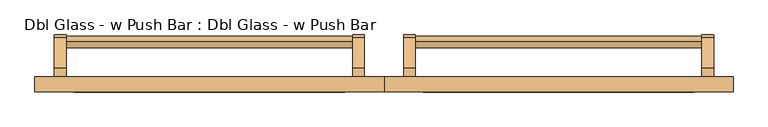
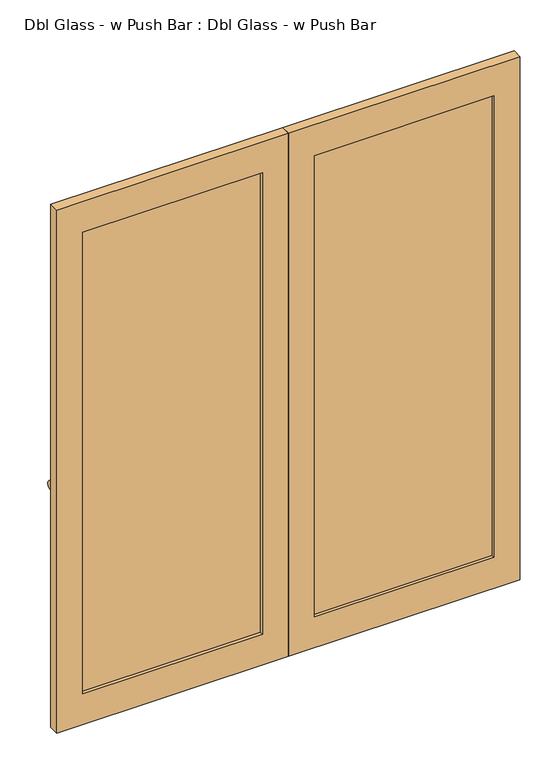
"""IFC4 building model written with IfcOpenShell, lengths in millimetres: door geometry, Dbl Glass - w Push Bar : Dbl Glass - w Push Bar."""

import ifcopenshell
import ifcopenshell.guid

model = None  # the IFC model being written
_history = None  # IfcOwnerHistory: only IFC2X3 demands one
_inside = {}  # id of a spatial element -> (the spatial element, [elements in it])
_under = {}  # id of a project, library or spatial element -> (it, [spatial elements below it])
_declared = {}  # id of a project -> (the project, [libraries it declares])
_typed = {}  # id of a type object -> (the type object, [elements of that type])
_made_of = {}  # id of a material, layer set ... -> (it, [elements and type objects made of it])


def new_model(schema):
    """Start an empty IFC model of exactly this schema.

    Asked for "IFC4X3", IfcOpenShell would pick the latest addendum, in which some entities
    have other attributes; the version numbers below select the first issue.
    IFC2X3 requires an IfcOwnerHistory on every rooted entity: one is made here for all.
    """
    global model, _history
    if schema == "IFC4X3":
        model = ifcopenshell.file(schema_version=(4, 3, 0, 0))
    else:
        model = ifcopenshell.file(schema=schema)
    _inside.clear()
    _under.clear()
    _declared.clear()
    _typed.clear()
    _made_of.clear()
    _history = None
    if model.schema == "IFC2X3":
        org = make("IfcOrganization", Name="unknown")
        user = make(
            "IfcPersonAndOrganization",
            ThePerson=make("IfcPerson", FamilyName="unknown"),
            TheOrganization=org,
        )
        app = make(
            "IfcApplication",
            ApplicationDeveloper=org,
            Version="unknown",
            ApplicationFullName="unknown",
            ApplicationIdentifier="unknown",
        )
        _history = make(
            "IfcOwnerHistory",
            OwningUser=user,
            OwningApplication=app,
            ChangeAction="ADDED",
            CreationDate=0,
        )
    return model


def make(cls, **values):
    """One entity of the class cls with the attributes given. An attribute that is None is left unset."""
    return model.create_entity(
        cls, **{name: value for name, value in values.items() if value is not None}
    )


def rooted(cls, **values):
    """An entity with a GlobalId (a new one), such as an element, a storey or a relation."""
    return make(cls, GlobalId=ifcopenshell.guid.new(), OwnerHistory=_history, **values)


def si_unit(unit_type, name, prefix=None):
    """IfcSIUnit, for example si_unit("LENGTHUNIT", "METRE", prefix="MILLI")."""
    return make("IfcSIUnit", UnitType=unit_type, Prefix=prefix, Name=name)


def assignment(units):
    """IfcUnitAssignment: the units of a project."""
    return None if units is None else make("IfcUnitAssignment", Units=units)


def point(xyz):
    """IfcCartesianPoint."""
    return None if xyz is None else make("IfcCartesianPoint", Coordinates=xyz)


def direction(xyz):
    """IfcDirection."""
    return None if xyz is None else make("IfcDirection", DirectionRatios=xyz)


def frame(location, z_axis=None, x_axis=None):
    """IfcAxis2Placement3D, a coordinate frame: its origin and axes. An axis left out is left unset."""
    return make(
        "IfcAxis2Placement3D",
        Location=point(location),
        Axis=direction(z_axis),
        RefDirection=direction(x_axis),
    )


def frame_2d(location, x_axis=None):
    """IfcAxis2Placement2D, a coordinate frame in the plane: its origin and x axis."""
    return make(
        "IfcAxis2Placement2D", Location=point(location), RefDirection=direction(x_axis)
    )


def origin():
    """The frame at (0, 0, 0) with its axes left unset."""
    return frame((0.0, 0.0, 0.0))


def place(relative_to, where):
    """IfcLocalPlacement: puts the frame where relative to a parent placement (None: the world)."""
    return make(
        "IfcLocalPlacement", PlacementRelTo=relative_to, RelativePlacement=where
    )


def context(
    kind, dimensions, precision=None, world=None, true_north=None, identifier=None
):
    """IfcGeometricRepresentationContext, for example the 3D "Model" context."""
    return make(
        "IfcGeometricRepresentationContext",
        ContextIdentifier=identifier,
        ContextType=kind,
        CoordinateSpaceDimension=dimensions,
        Precision=precision,
        WorldCoordinateSystem=world,
        TrueNorth=true_north,
    )


def project(units=None, contexts=None):
    """IfcProject with its units and contexts."""
    return rooted(
        "IfcProject",
        Name="project",
        RepresentationContexts=contexts,
        UnitsInContext=assignment(units),
    )


def spatial(cls, under=None, at=None, **own):
    """A site, building, storey or space (cls), placed at a placement, below another one or the project."""
    s = rooted(cls, ObjectPlacement=at, **own)
    if under is not None:
        _under.setdefault(under.id(), (under, []))[1].append(s)
    return s


def polyline(points):
    """IfcPolyline through the points."""
    return make("IfcPolyline", Points=[point(p) for p in points])


def circle_curve(where, radius):
    """IfcCircle in the frame where."""
    return make("IfcCircle", Position=where, Radius=radius)


def trimmed(basis, trim1, trim2, sense, master):
    """IfcTrimmedCurve: the piece of a basis curve between two trims."""
    return make(
        "IfcTrimmedCurve",
        BasisCurve=basis,
        Trim1=trim1,
        Trim2=trim2,
        SenseAgreement=sense,
        MasterRepresentation=master,
    )


def segment(curve, same_sense, transition):
    """IfcCompositeCurveSegment."""
    return make(
        "IfcCompositeCurveSegment",
        Transition=transition,
        SameSense=same_sense,
        ParentCurve=curve,
    )


def composite_curve(segments, self_intersect=None):
    """IfcCompositeCurve: segments joined end to end."""
    return make("IfcCompositeCurve", Segments=segments, SelfIntersect=self_intersect)


def outline(outer, holes=None, kind="AREA"):
    """IfcArbitraryClosedProfileDef: a profile drawn as a closed curve; with holes, ...WithVoids."""
    if holes is None:
        return make("IfcArbitraryClosedProfileDef", ProfileType=kind, OuterCurve=outer)
    return make(
        "IfcArbitraryProfileDefWithVoids",
        ProfileType=kind,
        OuterCurve=outer,
        InnerCurves=holes,
    )


def extrude(swept, where, along, depth):
    """IfcExtrudedAreaSolid: the profile swept, set in the frame where, extruded along a direction by depth."""
    return make(
        "IfcExtrudedAreaSolid",
        SweptArea=swept,
        Position=where,
        ExtrudedDirection=direction(along),
        Depth=depth,
    )


def shape(context_of_items, identifier, shape_type, items):
    """IfcShapeRepresentation: the items that make up one representation, for example the "Body"."""
    return make(
        "IfcShapeRepresentation",
        ContextOfItems=context_of_items,
        RepresentationIdentifier=identifier,
        RepresentationType=shape_type,
        Items=items,
    )


def source(mapping_origin, context_of_items, identifier, shape_type, items):
    """IfcRepresentationMap: a shape defined once, which mapped items show again and again."""
    return make(
        "IfcRepresentationMap",
        MappingOrigin=mapping_origin,
        MappedRepresentation=shape(context_of_items, identifier, shape_type, items),
    )


def transform(
    local_origin,
    x_axis=None,
    y_axis=None,
    z_axis=None,
    scale=None,
    scale2=None,
    scale3=None,
    uniform=True,
):
    """IfcCartesianTransformationOperator3D, or its non-uniform kind. x_axis, y_axis, z_axis: its Axis1, 2, 3."""
    if uniform:
        return make(
            "IfcCartesianTransformationOperator3D",
            Axis1=direction(x_axis),
            Axis2=direction(y_axis),
            LocalOrigin=point(local_origin),
            Scale=scale,
            Axis3=direction(z_axis),
        )
    return make(
        "IfcCartesianTransformationOperator3DnonUniform",
        Axis1=direction(x_axis),
        Axis2=direction(y_axis),
        LocalOrigin=point(local_origin),
        Scale=scale,
        Axis3=direction(z_axis),
        Scale2=scale2,
        Scale3=scale3,
    )


def mapped(mapping_source, mapping_target):
    """IfcMappedItem: shows the shape of a source again, moved by a transform."""
    return make(
        "IfcMappedItem", MappingSource=mapping_source, MappingTarget=mapping_target
    )


def made_of(thing, what):
    """Note that an element or type object is made of a material, layer set ...; save() writes the relation."""
    if what is not None:
        _made_of.setdefault(what.id(), (what, []))[1].append(thing)
    return thing


def element(
    cls,
    number,
    at=None,
    inside=None,
    cuts=None,
    type_object=None,
    material=None,
    context=None,
    identifier="Body",
    shape_type=None,
    held_by="IfcProductDefinitionShape",
    body=None,
    shapes=None,
    **own,
):
    """One element of the class cls, such as IfcWall. Its Tag is "e" and its number.

    at: its placement. inside: the storey or other place that contains it. cuts: it is an
    opening in that element (IfcRelVoidsElement). A single representation is given by context,
    identifier, shape_type and body (its items); several are given by shapes. held_by: the class
    of the entity that holds the representations. save() writes the other relations.
    """
    e = rooted(cls, Tag="e%d" % number, ObjectPlacement=at, **own)
    if body is not None:
        shapes = [shape(context, identifier, shape_type, body)]
    if shapes is not None:
        e.Representation = make(held_by, Representations=shapes)
    if inside is not None:
        _inside.setdefault(inside.id(), (inside, []))[1].append(e)
    if cuts is not None:
        rooted(
            "IfcRelVoidsElement", RelatingBuildingElement=cuts, RelatedOpeningElement=e
        )
    if type_object is not None:
        _typed.setdefault(type_object.id(), (type_object, []))[1].append(e)
    return made_of(e, material)


def aggregate(whole, parts):
    """IfcRelAggregates: a whole, such as a stair, and the parts it consists of."""
    return rooted("IfcRelAggregates", RelatingObject=whole, RelatedObjects=parts)


def save(model, path):
    """Write the relations noted so far, then the file.

    IfcRelAggregates (storeys below a building ...), IfcRelContainedInSpatialStructure (elements
    in a storey), IfcRelDefinesByType, IfcRelAssociatesMaterial and IfcRelDeclares: one each for
    every whole, place, type object, material and project.
    """
    for whole, parts in _under.values():
        aggregate(whole, parts)
    for where, things in _inside.values():
        rooted(
            "IfcRelContainedInSpatialStructure",
            RelatedElements=things,
            RelatingStructure=where,
        )
    for kind, things in _typed.values():
        rooted("IfcRelDefinesByType", RelatedObjects=things, RelatingType=kind)
    for what, things in _made_of.values():
        rooted("IfcRelAssociatesMaterial", RelatedObjects=things, RelatingMaterial=what)
    for by, libraries in _declared.values():
        rooted("IfcRelDeclares", RelatingContext=by, RelatedDefinitions=libraries)
    model.write(path)


def dbl_glass_w_push_bar_dbl_glass_w_push_bar_b5e52d6e(model_context):
    return source(origin(), model_context, "Body", "SweptSolid", [
        extrude(outline(composite_curve([segment(trimmed(circle_curve(frame_2d((65.0203019, 909.5721086)), 15.0), [point((65.0203019, 924.5721086))], [point((65.0203019, 894.5721086))], False, "CARTESIAN"), True, "CONTINUOUS"), segment(trimmed(circle_curve(frame_2d((65.0203019, 909.5721086)), 15.0), [point((65.0203019, 894.5721086))], [point((65.0203019, 924.5721086))], False, "CARTESIAN"), True, "CONTINUOUS")], self_intersect=False)), frame((80.0, 0.0, 0.0), z_axis=(1.0, 0.0, 0.0), x_axis=(0.0, 1.0, 0.0)), (0.0, 0.0, 1.0), 731.0),
        extrude(outline(composite_curve([segment(polyline([(-0.1563269, 1000.0), (77.6459332, 922.19774)]), True, "CONTINUOUS"), segment(trimmed(circle_curve(frame_2d((65.0203019, 909.5721086)), 17.8553391), [point((77.6459332, 922.19774))], [point((52.3946705, 896.9464773))], False, "CARTESIAN"), True, "CONTINUOUS"), segment(polyline([(52.3946705, 896.9464773), (14.3411478, 935.0), (-24.035259, 935.0), (-24.035259, 1000.0), (-0.1563269, 1000.0)]), True, "CONTINUOUS")], self_intersect=False)), frame((811.0, 0.0, 0.0), z_axis=(1.0, 0.0, 0.0), x_axis=(0.0, 1.0, 0.0)), (0.0, 0.0, 1.0), 30.0),
        extrude(outline(composite_curve([segment(polyline([(-0.1563269, 1000.0), (77.6459332, 922.19774)]), True, "CONTINUOUS"), segment(trimmed(circle_curve(frame_2d((65.0203019, 909.5721086)), 17.8553391), [point((77.6459332, 922.19774))], [point((52.3946705, 896.9464773))], False, "CARTESIAN"), True, "CONTINUOUS"), segment(polyline([(52.3946705, 896.9464773), (14.3411478, 935.0), (-24.035259, 935.0), (-24.035259, 1000.0), (-0.1563269, 1000.0)]), True, "CONTINUOUS")], self_intersect=False)), frame((50.0, 0.0, 0.0), z_axis=(1.0, 0.0, 0.0), x_axis=(0.0, 1.0, 0.0)), (0.0, 0.0, 1.0), 30.0),
        extrude(outline(composite_curve([segment(trimmed(circle_curve(frame_2d((65.0203019, 909.5721086)), 15.0), [point((65.0203019, 924.5721086))], [point((65.0203019, 894.5721086))], False, "CARTESIAN"), True, "CONTINUOUS"), segment(trimmed(circle_curve(frame_2d((65.0203019, 909.5721086)), 15.0), [point((65.0203019, 894.5721086))], [point((65.0203019, 924.5721086))], False, "CARTESIAN"), True, "CONTINUOUS")], self_intersect=False)), frame((-811.0, 0.0, 0.0), z_axis=(1.0, 0.0, 0.0), x_axis=(0.0, 1.0, 0.0)), (0.0, 0.0, 1.0), 731.0),
        extrude(outline(composite_curve([segment(polyline([(-0.1563269, 1000.0), (77.6459332, 922.19774)]), True, "CONTINUOUS"), segment(trimmed(circle_curve(frame_2d((65.0203019, 909.5721086)), 17.8553391), [point((77.6459332, 922.19774))], [point((52.3946705, 896.9464773))], False, "CARTESIAN"), True, "CONTINUOUS"), segment(polyline([(52.3946705, 896.9464773), (14.3411478, 935.0), (-24.035259, 935.0), (-24.035259, 1000.0), (-0.1563269, 1000.0)]), True, "CONTINUOUS")], self_intersect=False)), frame((-80.0, 0.0, 0.0), z_axis=(1.0, 0.0, 0.0), x_axis=(0.0, 1.0, 0.0)), (0.0, 0.0, 1.0), 30.0),
        extrude(outline(composite_curve([segment(polyline([(-0.1563269, 1000.0), (77.6459332, 922.19774)]), True, "CONTINUOUS"), segment(trimmed(circle_curve(frame_2d((65.0203019, 909.5721086)), 17.8553391), [point((77.6459332, 922.19774))], [point((52.3946705, 896.9464773))], False, "CARTESIAN"), True, "CONTINUOUS"), segment(polyline([(52.3946705, 896.9464773), (14.3411478, 935.0), (-24.035259, 935.0), (-24.035259, 1000.0), (-0.1563269, 1000.0)]), True, "CONTINUOUS")], self_intersect=False)), frame((-841.0, 0.0, 0.0), z_axis=(1.0, 0.0, 0.0), x_axis=(0.0, 1.0, 0.0)), (0.0, 0.0, 1.0), 30.0),
        extrude(outline(polyline([(2125.0, -891.0), (0.0, -891.0), (0.0, 0.0), (2125.0, 0.0), (2125.0, -891.0)]), holes=[polyline([(2000.0, -791.0), (2000.0, -100.0), (125.0, -100.0), (125.0, -791.0), (2000.0, -791.0)])]), frame((0.0, -62.5788556, 0.0), z_axis=(0.0, 1.0, 0.0), x_axis=(0.0, 0.0, 1.0)), (0.0, 0.0, 1.0), 38.5435966),
        extrude(outline(polyline([(2125.0, 0.0), (0.0, 0.0), (0.0, 891.0), (2125.0, 891.0), (2125.0, 0.0)]), holes=[polyline([(2000.0, 100.0), (2000.0, 791.0), (125.0, 791.0), (125.0, 100.0), (2000.0, 100.0)])]), frame((0.0, -62.5788556, 0.0), z_axis=(0.0, 1.0, 0.0), x_axis=(0.0, 0.0, 1.0)), (0.0, 0.0, 1.0), 38.5435966),
        extrude(outline(polyline([(-100.0, -38.0), (-100.0, -50.0), (-791.0, -50.0), (-791.0, -38.0), (-100.0, -38.0)])), frame((0.0, 0.0, 125.0), z_axis=(0.0, 0.0, 1.0), x_axis=(1.0, 0.0, 0.0)), (0.0, 0.0, 1.0), 1875.0),
        extrude(outline(polyline([(791.0, -38.0), (791.0, -50.0), (100.0, -50.0), (100.0, -38.0), (791.0, -38.0)])), frame((0.0, 0.0, 125.0), z_axis=(0.0, 0.0, 1.0), x_axis=(1.0, 0.0, 0.0)), (0.0, 0.0, 1.0), 1875.0),
    ])


if __name__ == "__main__":
    model = new_model("IFC4")
    model_context = context("Model", 3, world=origin())
    ifc_project = project(units=[si_unit("LENGTHUNIT", "METRE", prefix="MILLI")], contexts=[model_context])
    site = spatial("IfcSite", under=ifc_project)
    building = spatial("IfcBuilding", under=site)
    placement = place(None, origin())
    dbl_glass_w_push_bar_dbl_glass_w_push_bar_shape = dbl_glass_w_push_bar_dbl_glass_w_push_bar_b5e52d6e(model_context)
    element("IfcDoor", 1, ObjectType="Dbl Glass - w Push Bar : Dbl Glass - w Push Bar", at=placement, inside=building, context=model_context, shape_type="MappedRepresentation", body=[
        mapped(dbl_glass_w_push_bar_dbl_glass_w_push_bar_shape, transform((0.0, 0.0, 0.0), x_axis=(1.0, 0.0, 0.0), y_axis=(0.0, 1.0, 0.0), z_axis=(0.0, 0.0, 1.0))),
    ])
    save(model, "model.ifc")

# Revit data of these elements
# Type "Dbl Glass - w Push Bar : Dbl Glass - w Push Bar"
#   Description = "Curtain Wall Door"
#   Type Mark = "55"
#   Construction Type Id = "GSP4R"
#   Analytic Construction = "1/8 in Pilkington single glazing"
#   Visual Light Transmittance = 0.9
#   TopRail = 125 mm
#   Solar Heat Gain Coefficient = 0.78
#   Offset = 50 mm
#   MuntinRail = 100 mm
#   LockRail = 100 mm
#   Heat Transfer Coefficient (U) = 3.6886 W/(m²·K)
#   Handle Z Distance = 1000 mm
#   Handle X Offset = 65 mm
#   Glass Thickness = 12 mm
#   BottomRail = 125 mm
#   Define Thermal Properties by = 1
#   Material Ironmongery = Metal - Aluminum
#   Material Door = Metal - Aluminum
#   Material Glass = Glass
#   Function = (empty or 0)
# Element 1 (IfcDoor, "Dbl Glass - w Push Bar : Dbl Glass - w Push Bar")
#   Materials on its faces: "Metal - Aluminum", "Glass"
# Materials
#   "Metal - Aluminum": class "Metal", colour RGB 247 247 247, transparency 0
#   "Glass": class "Glass", colour RGB 0 128 192, transparency 0.9, Description = "Soda Lime Glass", Cost = 0
